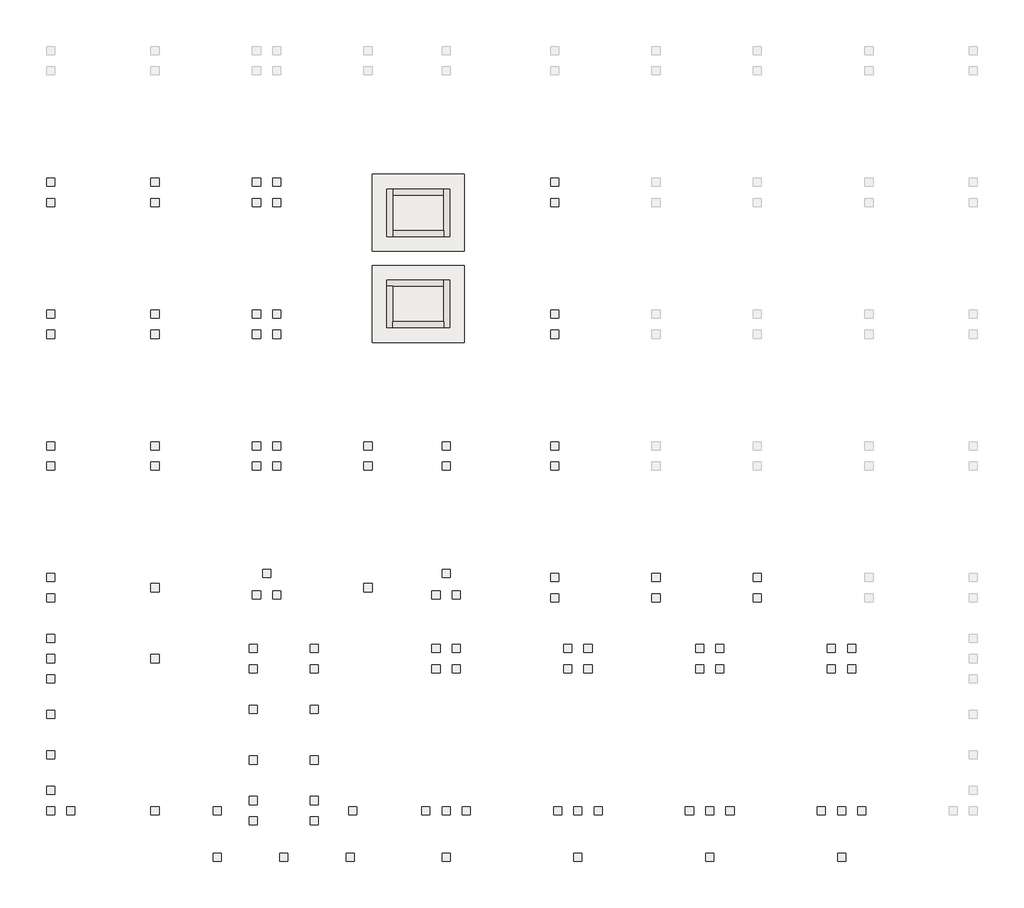
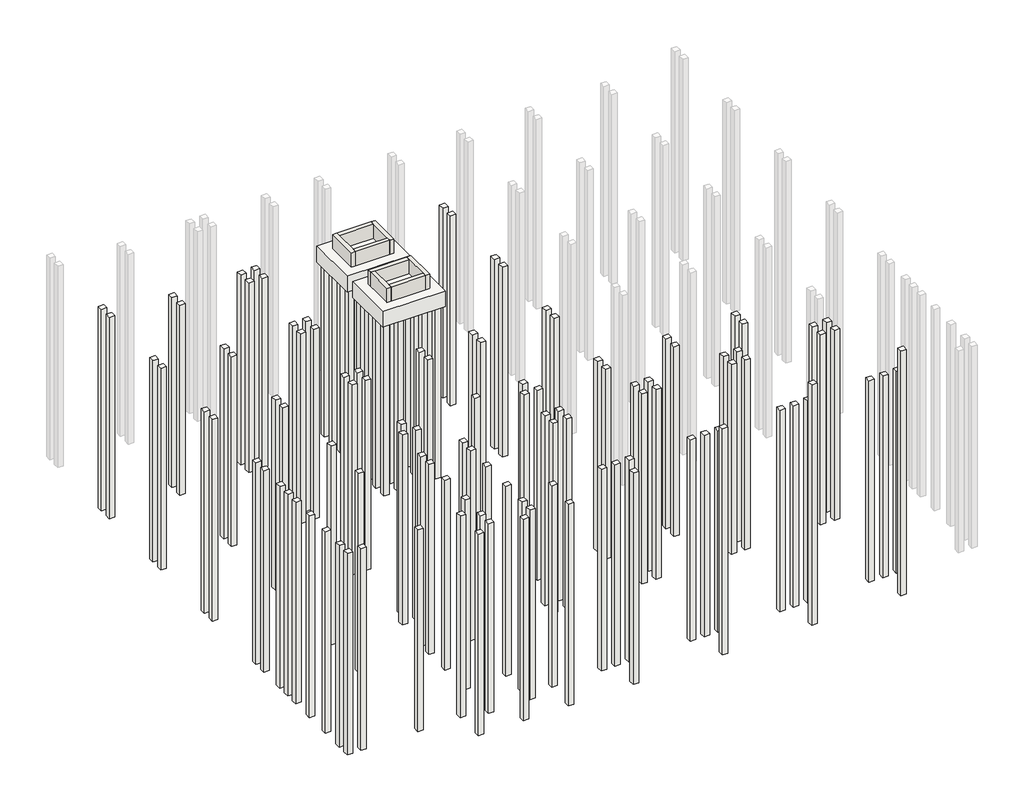
# Not in any storey, part 1 of 2: 143 footings, 8 walls.
"""IFC4 building model written with IfcOpenShell, lengths in millimetres."""

import ifcopenshell
import ifcopenshell.guid

model = None  # the IFC model being written
_history = None  # IfcOwnerHistory: only IFC2X3 demands one
_inside = {}  # id of a spatial element -> (the spatial element, [elements in it])
_under = {}  # id of a project, library or spatial element -> (it, [spatial elements below it])
_declared = {}  # id of a project -> (the project, [libraries it declares])
_typed = {}  # id of a type object -> (the type object, [elements of that type])
_made_of = {}  # id of a material, layer set ... -> (it, [elements and type objects made of it])


def new_model(schema):
    """Start an empty IFC model of exactly this schema.

    Asked for "IFC4X3", IfcOpenShell would pick the latest addendum, in which some entities
    have other attributes; the version numbers below select the first issue.
    IFC2X3 requires an IfcOwnerHistory on every rooted entity: one is made here for all.
    """
    global model, _history
    if schema == "IFC4X3":
        model = ifcopenshell.file(schema_version=(4, 3, 0, 0))
    else:
        model = ifcopenshell.file(schema=schema)
    _inside.clear()
    _under.clear()
    _declared.clear()
    _typed.clear()
    _made_of.clear()
    _history = None
    if model.schema == "IFC2X3":
        org = make("IfcOrganization", Name="unknown")
        user = make(
            "IfcPersonAndOrganization",
            ThePerson=make("IfcPerson", FamilyName="unknown"),
            TheOrganization=org,
        )
        app = make(
            "IfcApplication",
            ApplicationDeveloper=org,
            Version="unknown",
            ApplicationFullName="unknown",
            ApplicationIdentifier="unknown",
        )
        _history = make(
            "IfcOwnerHistory",
            OwningUser=user,
            OwningApplication=app,
            ChangeAction="ADDED",
            CreationDate=0,
        )
    return model


def make(cls, **values):
    """One entity of the class cls with the attributes given. An attribute that is None is left unset."""
    return model.create_entity(
        cls, **{name: value for name, value in values.items() if value is not None}
    )


def rooted(cls, **values):
    """An entity with a GlobalId (a new one), such as an element, a storey or a relation."""
    return make(cls, GlobalId=ifcopenshell.guid.new(), OwnerHistory=_history, **values)


def si_unit(unit_type, name, prefix=None):
    """IfcSIUnit, for example si_unit("LENGTHUNIT", "METRE", prefix="MILLI")."""
    return make("IfcSIUnit", UnitType=unit_type, Prefix=prefix, Name=name)


def assignment(units):
    """IfcUnitAssignment: the units of a project."""
    return None if units is None else make("IfcUnitAssignment", Units=units)


def point(xyz):
    """IfcCartesianPoint."""
    return None if xyz is None else make("IfcCartesianPoint", Coordinates=xyz)


def direction(xyz):
    """IfcDirection."""
    return None if xyz is None else make("IfcDirection", DirectionRatios=xyz)


def frame(location, z_axis=None, x_axis=None):
    """IfcAxis2Placement3D, a coordinate frame: its origin and axes. An axis left out is left unset."""
    return make(
        "IfcAxis2Placement3D",
        Location=point(location),
        Axis=direction(z_axis),
        RefDirection=direction(x_axis),
    )


def origin():
    """The frame at (0, 0, 0) with its axes left unset."""
    return frame((0.0, 0.0, 0.0))


def place(relative_to, where):
    """IfcLocalPlacement: puts the frame where relative to a parent placement (None: the world)."""
    return make(
        "IfcLocalPlacement", PlacementRelTo=relative_to, RelativePlacement=where
    )


def context(
    kind, dimensions, precision=None, world=None, true_north=None, identifier=None
):
    """IfcGeometricRepresentationContext, for example the 3D "Model" context."""
    return make(
        "IfcGeometricRepresentationContext",
        ContextIdentifier=identifier,
        ContextType=kind,
        CoordinateSpaceDimension=dimensions,
        Precision=precision,
        WorldCoordinateSystem=world,
        TrueNorth=true_north,
    )


def project(units=None, contexts=None):
    """IfcProject with its units and contexts."""
    return rooted(
        "IfcProject",
        Name="project",
        RepresentationContexts=contexts,
        UnitsInContext=assignment(units),
    )


def spatial(cls, under=None, at=None, **own):
    """A site, building, storey or space (cls), placed at a placement, below another one or the project."""
    s = rooted(cls, ObjectPlacement=at, **own)
    if under is not None:
        _under.setdefault(under.id(), (under, []))[1].append(s)
    return s


def polyline(points):
    """IfcPolyline through the points."""
    return make("IfcPolyline", Points=[point(p) for p in points])


def outline(outer, holes=None, kind="AREA"):
    """IfcArbitraryClosedProfileDef: a profile drawn as a closed curve; with holes, ...WithVoids."""
    if holes is None:
        return make("IfcArbitraryClosedProfileDef", ProfileType=kind, OuterCurve=outer)
    return make(
        "IfcArbitraryProfileDefWithVoids",
        ProfileType=kind,
        OuterCurve=outer,
        InnerCurves=holes,
    )


def extrude(swept, where, along, depth):
    """IfcExtrudedAreaSolid: the profile swept, set in the frame where, extruded along a direction by depth."""
    return make(
        "IfcExtrudedAreaSolid",
        SweptArea=swept,
        Position=where,
        ExtrudedDirection=direction(along),
        Depth=depth,
    )


def faces_of(points, faces, orient=None, outer=None):
    """IfcFace entities. A face is a list of loops; a loop is a list of indices into points, from 0.

    orient and outer hold one flag for each loop. By default every Orientation is true, the
    first loop of a face is its IfcFaceOuterBound and the others are IfcFaceBound.
    """
    made = []
    for i, loops in enumerate(faces):
        bounds = []
        for j, loop in enumerate(loops):
            is_outer = j == 0 if outer is None else outer[i][j]
            bounds.append(
                make(
                    "IfcFaceOuterBound" if is_outer else "IfcFaceBound",
                    Bound=make("IfcPolyLoop", Polygon=[points[k] for k in loop]),
                    Orientation=True if orient is None else orient[i][j],
                )
            )
        made.append(make("IfcFace", Bounds=bounds))
    return made


def faceted_brep(points, faces, orient=None, outer=None, voids=None):
    """IfcFacetedBrep: a solid bounded by flat faces; with voids (closed shells), ...WithVoids."""
    shared = [point(p) for p in points]
    hull = make("IfcClosedShell", CfsFaces=faces_of(shared, faces, orient, outer))
    if voids is None:
        return make("IfcFacetedBrep", Outer=hull)
    return make(
        "IfcFacetedBrepWithVoids",
        Outer=hull,
        Voids=[
            make(cls, CfsFaces=faces_of(shared, fs, o, b)) for cls, fs, o, b in voids
        ],
    )


def shape(context_of_items, identifier, shape_type, items):
    """IfcShapeRepresentation: the items that make up one representation, for example the "Body"."""
    return make(
        "IfcShapeRepresentation",
        ContextOfItems=context_of_items,
        RepresentationIdentifier=identifier,
        RepresentationType=shape_type,
        Items=items,
    )


def source(mapping_origin, context_of_items, identifier, shape_type, items):
    """IfcRepresentationMap: a shape defined once, which mapped items show again and again."""
    return make(
        "IfcRepresentationMap",
        MappingOrigin=mapping_origin,
        MappedRepresentation=shape(context_of_items, identifier, shape_type, items),
    )


def transform(
    local_origin,
    x_axis=None,
    y_axis=None,
    z_axis=None,
    scale=None,
    scale2=None,
    scale3=None,
    uniform=True,
):
    """IfcCartesianTransformationOperator3D, or its non-uniform kind. x_axis, y_axis, z_axis: its Axis1, 2, 3."""
    if uniform:
        return make(
            "IfcCartesianTransformationOperator3D",
            Axis1=direction(x_axis),
            Axis2=direction(y_axis),
            LocalOrigin=point(local_origin),
            Scale=scale,
            Axis3=direction(z_axis),
        )
    return make(
        "IfcCartesianTransformationOperator3DnonUniform",
        Axis1=direction(x_axis),
        Axis2=direction(y_axis),
        LocalOrigin=point(local_origin),
        Scale=scale,
        Axis3=direction(z_axis),
        Scale2=scale2,
        Scale3=scale3,
    )


def mapped(mapping_source, mapping_target):
    """IfcMappedItem: shows the shape of a source again, moved by a transform."""
    return make(
        "IfcMappedItem", MappingSource=mapping_source, MappingTarget=mapping_target
    )


def made_of(thing, what):
    """Note that an element or type object is made of a material, layer set ...; save() writes the relation."""
    if what is not None:
        _made_of.setdefault(what.id(), (what, []))[1].append(thing)
    return thing


def element(
    cls,
    number,
    at=None,
    inside=None,
    cuts=None,
    type_object=None,
    material=None,
    context=None,
    identifier="Body",
    shape_type=None,
    held_by="IfcProductDefinitionShape",
    body=None,
    shapes=None,
    **own,
):
    """One element of the class cls, such as IfcWall. Its Tag is "e" and its number.

    at: its placement. inside: the storey or other place that contains it. cuts: it is an
    opening in that element (IfcRelVoidsElement). A single representation is given by context,
    identifier, shape_type and body (its items); several are given by shapes. held_by: the class
    of the entity that holds the representations. save() writes the other relations.
    """
    e = rooted(cls, Tag="e%d" % number, ObjectPlacement=at, **own)
    if body is not None:
        shapes = [shape(context, identifier, shape_type, body)]
    if shapes is not None:
        e.Representation = make(held_by, Representations=shapes)
    if inside is not None:
        _inside.setdefault(inside.id(), (inside, []))[1].append(e)
    if cuts is not None:
        rooted(
            "IfcRelVoidsElement", RelatingBuildingElement=cuts, RelatedOpeningElement=e
        )
    if type_object is not None:
        _typed.setdefault(type_object.id(), (type_object, []))[1].append(e)
    return made_of(e, material)


def aggregate(whole, parts):
    """IfcRelAggregates: a whole, such as a stair, and the parts it consists of."""
    return rooted("IfcRelAggregates", RelatingObject=whole, RelatedObjects=parts)


def save(model, path):
    """Write the relations noted so far, then the file.

    IfcRelAggregates (storeys below a building ...), IfcRelContainedInSpatialStructure (elements
    in a storey), IfcRelDefinesByType, IfcRelAssociatesMaterial and IfcRelDeclares: one each for
    every whole, place, type object, material and project.
    """
    for whole, parts in _under.values():
        aggregate(whole, parts)
    for where, things in _inside.values():
        rooted(
            "IfcRelContainedInSpatialStructure",
            RelatedElements=things,
            RelatingStructure=where,
        )
    for kind, things in _typed.values():
        rooted("IfcRelDefinesByType", RelatedObjects=things, RelatingType=kind)
    for what, things in _made_of.values():
        rooted("IfcRelAssociatesMaterial", RelatedObjects=things, RelatingMaterial=what)
    for by, libraries in _declared.values():
        rooted("IfcRelDeclares", RelatingContext=by, RelatedDefinitions=libraries)
    model.write(path)


def footing_e3f33549(model_context):
    return source(origin(), model_context, "Body", "SweptSolid", [
        extrude(outline(polyline([(200.0, -200.0), (-200.0, -200.0), (-200.0, 200.0), (200.0, 200.0), (200.0, -200.0)])), frame((0.0, 0.0, -20000.0), z_axis=(0.0, 0.0, 1.0), x_axis=(1.0, 0.0, 0.0)), (0.0, 0.0, 1.0), 15320.0),
    ])


def footing_2462c6b3(model_context):
    return source(origin(), model_context, "Body", "SweptSolid", [
        extrude(outline(polyline([(200.0, -200.0), (-200.0, -200.0), (-200.0, 200.0), (200.0, 200.0), (200.0, -200.0)])), frame((0.0, 0.0, -20000.0), z_axis=(0.0, 0.0, 1.0), x_axis=(1.0, 0.0, 0.0)), (0.0, 0.0, 1.0), 14620.0),
    ])


def footing_4eaa82be(model_context):
    return source(origin(), model_context, "Body", "SweptSolid", [
        extrude(outline(polyline([(200.0, -200.0), (-200.0, -200.0), (-200.0, 200.0), (200.0, 200.0), (200.0, -200.0)])), frame((0.0, 0.0, -20000.0), z_axis=(0.0, 0.0, 1.0), x_axis=(1.0, 0.0, 0.0)), (0.0, 0.0, 1.0), 15520.0),
    ])


def footing_98706cf3(model_context):
    return source(origin(), model_context, "Body", "SweptSolid", [
        extrude(outline(polyline([(200.0, -200.0), (-200.0, -200.0), (-200.0, 200.0), (200.0, 200.0), (200.0, -200.0)])), frame((0.0, 0.0, -20000.0), z_axis=(0.0, 0.0, 1.0), x_axis=(1.0, 0.0, 0.0)), (0.0, 0.0, 1.0), 16280.0),
    ])


def footing_73a1868d(model_context):
    return source(origin(), model_context, "Body", "SweptSolid", [
        extrude(outline(polyline([(200.0, -200.0), (-200.0, -200.0), (-200.0, 200.0), (200.0, 200.0), (200.0, -200.0)])), frame((0.0, 0.0, -20000.0), z_axis=(0.0, 0.0, 1.0), x_axis=(1.0, 0.0, 0.0)), (0.0, 0.0, 1.0), 17400.0),
    ])


def footing_81e4ded3(model_context):
    return source(origin(), model_context, "Body", "SweptSolid", [
        extrude(outline(polyline([(200.0, -200.0), (-200.0, -200.0), (-200.0, 200.0), (200.0, 200.0), (200.0, -200.0)])), frame((0.0, 0.0, -20000.0), z_axis=(0.0, 0.0, 1.0), x_axis=(1.0, 0.0, 0.0)), (0.0, 0.0, 1.0), 18520.0),
    ])


def footing_0d914d5e(model_context):
    return source(origin(), model_context, "Body", "SweptSolid", [
        extrude(outline(polyline([(200.0, -200.0), (-200.0, -200.0), (-200.0, 200.0), (200.0, 200.0), (200.0, -200.0)])), frame((0.0, 0.0, -20000.0), z_axis=(0.0, 0.0, 1.0), x_axis=(1.0, 0.0, 0.0)), (0.0, 0.0, 1.0), 18850.0),
    ])


def footing_443494b9(model_context):
    return source(origin(), model_context, "Body", "SweptSolid", [
        extrude(outline(polyline([(200.0, -200.0), (-200.0, -200.0), (-200.0, 200.0), (200.0, 200.0), (200.0, -200.0)])), frame((0.0, 0.0, -20000.0), z_axis=(0.0, 0.0, 1.0), x_axis=(1.0, 0.0, 0.0)), (0.0, 0.0, 1.0), 13220.0),
    ])


model = new_model("IFC4")

# Units and contexts
model_context = context("Model", 3, world=origin())
ifc_project = project(units=[si_unit("LENGTHUNIT", "METRE", prefix="MILLI")], contexts=[model_context])

# Site, building
site = spatial("IfcSite", under=ifc_project)
building = spatial("IfcBuilding", under=site)

# Footings
placement = place(None, origin())
element("IfcFooting", 1, at=placement, inside=building, context=model_context, shape_type="SweptSolid", body=[
    extrude(outline(polyline([(22350.0, 27600.0), (22350.0, 31400.0), (26900.0, 31400.0), (26900.0, 27600.0), (22350.0, 27600.0)])), frame((0.0, 0.0, -6800.0), z_axis=(0.0, 0.0, 1.0), x_axis=(1.0, 0.0, 0.0)), (0.0, 0.0, 1.0), 1200.0),
])
element("IfcFooting", 2, at=placement, inside=building, context=model_context, shape_type="SweptSolid", body=[
    extrude(outline(polyline([(22350.0, 23100.0), (22350.0, 26900.0), (26900.0, 26900.0), (26900.0, 23100.0), (22350.0, 23100.0)])), frame((0.0, 0.0, -6800.0), z_axis=(0.0, 0.0, 1.0), x_axis=(1.0, 0.0, 0.0)), (0.0, 0.0, 1.0), 1200.0),
])
footing_shape = footing_e3f33549(model_context)
element("IfcFooting", 3, at=placement, inside=building, context=model_context, shape_type="MappedRepresentation", body=[
    mapped(footing_shape, transform((11650.0, 7500.0, 0.0), x_axis=(1.0, 0.0, 0.0), y_axis=(0.0, 1.0, 0.0), z_axis=(0.0, 0.0, 1.0))),
])
element("IfcFooting", 4, at=placement, inside=building, context=model_context, shape_type="MappedRepresentation", body=[
    mapped(footing_shape, transform((11650.0, 11000.0, 0.0), x_axis=(1.0, 0.0, 0.0), y_axis=(0.0, 1.0, 0.0), z_axis=(0.0, 0.0, 1.0))),
])
element("IfcFooting", 5, at=placement, inside=building, context=model_context, shape_type="MappedRepresentation", body=[
    mapped(footing_shape, transform((22150.0, 11000.0, 0.0), x_axis=(1.0, 0.0, 0.0), y_axis=(0.0, 1.0, 0.0), z_axis=(0.0, 0.0, 1.0))),
])
footing_2_shape = footing_2462c6b3(model_context)
element("IfcFooting", 6, at=placement, inside=building, context=model_context, shape_type="MappedRepresentation", body=[
    mapped(footing_2_shape, transform((22150.0, 17000.0, 0.0), x_axis=(1.0, 0.0, 0.0), y_axis=(0.0, 1.0, 0.0), z_axis=(0.0, 0.0, 1.0))),
])
element("IfcFooting", 7, at=placement, inside=building, context=model_context, shape_type="MappedRepresentation", body=[
    mapped(footing_2_shape, transform((22150.0, 18000.0, 0.0), x_axis=(1.0, 0.0, 0.0), y_axis=(0.0, 1.0, 0.0), z_axis=(0.0, 0.0, 1.0))),
])
element("IfcFooting", 8, at=placement, inside=building, context=model_context, shape_type="MappedRepresentation", body=[
    mapped(footing_2_shape, transform((26000.0, 17000.0, 0.0), x_axis=(1.0, 0.0, 0.0), y_axis=(0.0, 1.0, 0.0), z_axis=(0.0, 0.0, 1.0))),
])
element("IfcFooting", 9, at=placement, inside=building, context=model_context, shape_type="MappedRepresentation", body=[
    mapped(footing_2_shape, transform((26000.0, 18000.0, 0.0), x_axis=(1.0, 0.0, 0.0), y_axis=(0.0, 1.0, 0.0), z_axis=(0.0, 0.0, 1.0))),
])
element("IfcFooting", 10, at=placement, inside=building, context=model_context, shape_type="MappedRepresentation", body=[
    mapped(footing_2_shape, transform((11650.0, 17000.0, 0.0), x_axis=(1.0, 0.0, 0.0), y_axis=(0.0, 1.0, 0.0), z_axis=(0.0, 0.0, 1.0))),
])
element("IfcFooting", 11, at=placement, inside=building, context=model_context, shape_type="MappedRepresentation", body=[
    mapped(footing_2_shape, transform((11650.0, 18000.0, 0.0), x_axis=(1.0, 0.0, 0.0), y_axis=(0.0, 1.0, 0.0), z_axis=(0.0, 0.0, 1.0))),
])
element("IfcFooting", 12, at=placement, inside=building, context=model_context, shape_type="MappedRepresentation", body=[
    mapped(footing_2_shape, transform((11650.0, 23500.0, 0.0), x_axis=(1.0, 0.0, 0.0), y_axis=(0.0, 1.0, 0.0), z_axis=(0.0, 0.0, 1.0))),
])
element("IfcFooting", 13, at=placement, inside=building, context=model_context, shape_type="MappedRepresentation", body=[
    mapped(footing_2_shape, transform((11650.0, 24500.0, 0.0), x_axis=(1.0, 0.0, 0.0), y_axis=(0.0, 1.0, 0.0), z_axis=(0.0, 0.0, 1.0))),
])
element("IfcFooting", 14, at=placement, inside=building, context=model_context, shape_type="MappedRepresentation", body=[
    mapped(footing_2_shape, transform((11650.0, 30000.0, 0.0), x_axis=(1.0, 0.0, 0.0), y_axis=(0.0, 1.0, 0.0), z_axis=(0.0, 0.0, 1.0))),
])
element("IfcFooting", 15, at=placement, inside=building, context=model_context, shape_type="MappedRepresentation", body=[
    mapped(footing_2_shape, transform((11650.0, 31000.0, 0.0), x_axis=(1.0, 0.0, 0.0), y_axis=(0.0, 1.0, 0.0), z_axis=(0.0, 0.0, 1.0))),
])
element("IfcFooting", 16, at=placement, inside=building, context=model_context, shape_type="MappedRepresentation", body=[
    mapped(footing_2_shape, transform((31350.0, 10500.0, 0.0), x_axis=(1.0, 0.0, 0.0), y_axis=(0.0, 1.0, 0.0), z_axis=(0.0, 0.0, 1.0))),
])
element("IfcFooting", 17, at=placement, inside=building, context=model_context, shape_type="MappedRepresentation", body=[
    mapped(footing_2_shape, transform((31350.0, 11500.0, 0.0), x_axis=(1.0, 0.0, 0.0), y_axis=(0.0, 1.0, 0.0), z_axis=(0.0, 0.0, 1.0))),
])
element("IfcFooting", 18, at=placement, inside=building, context=model_context, shape_type="MappedRepresentation", body=[
    mapped(footing_2_shape, transform((36350.0, 10500.0, 0.0), x_axis=(1.0, 0.0, 0.0), y_axis=(0.0, 1.0, 0.0), z_axis=(0.0, 0.0, 1.0))),
])
element("IfcFooting", 19, at=placement, inside=building, context=model_context, shape_type="MappedRepresentation", body=[
    mapped(footing_2_shape, transform((36350.0, 11500.0, 0.0), x_axis=(1.0, 0.0, 0.0), y_axis=(0.0, 1.0, 0.0), z_axis=(0.0, 0.0, 1.0))),
])
element("IfcFooting", 20, at=placement, inside=building, context=model_context, shape_type="MappedRepresentation", body=[
    mapped(footing_2_shape, transform((41350.0, 10500.0, 0.0), x_axis=(1.0, 0.0, 0.0), y_axis=(0.0, 1.0, 0.0), z_axis=(0.0, 0.0, 1.0))),
])
element("IfcFooting", 21, at=placement, inside=building, context=model_context, shape_type="MappedRepresentation", body=[
    mapped(footing_2_shape, transform((41350.0, 11500.0, 0.0), x_axis=(1.0, 0.0, 0.0), y_axis=(0.0, 1.0, 0.0), z_axis=(0.0, 0.0, 1.0))),
])
element("IfcFooting", 22, at=placement, inside=building, context=model_context, shape_type="MappedRepresentation", body=[
    mapped(footing_2_shape, transform((46000.0, 7000.0, 0.0), x_axis=(1.0, 0.0, 0.0), y_axis=(0.0, 1.0, 0.0), z_axis=(0.0, 0.0, 1.0))),
])
element("IfcFooting", 23, at=placement, inside=building, context=model_context, shape_type="MappedRepresentation", body=[
    mapped(footing_2_shape, transform((46000.0, 8000.0, 0.0), x_axis=(1.0, 0.0, 0.0), y_axis=(0.0, 1.0, 0.0), z_axis=(0.0, 0.0, 1.0))),
])
element("IfcFooting", 24, at=placement, inside=building, context=model_context, shape_type="MappedRepresentation", body=[
    mapped(footing_2_shape, transform((45000.0, 7000.0, 0.0), x_axis=(1.0, 0.0, 0.0), y_axis=(0.0, 1.0, 0.0), z_axis=(0.0, 0.0, 1.0))),
])
element("IfcFooting", 25, at=placement, inside=building, context=model_context, shape_type="MappedRepresentation", body=[
    mapped(footing_2_shape, transform((45000.0, 8000.0, 0.0), x_axis=(1.0, 0.0, 0.0), y_axis=(0.0, 1.0, 0.0), z_axis=(0.0, 0.0, 1.0))),
])
element("IfcFooting", 26, at=placement, inside=building, context=model_context, shape_type="MappedRepresentation", body=[
    mapped(footing_2_shape, transform((39500.0, 7000.0, 0.0), x_axis=(1.0, 0.0, 0.0), y_axis=(0.0, 1.0, 0.0), z_axis=(0.0, 0.0, 1.0))),
])
element("IfcFooting", 27, at=placement, inside=building, context=model_context, shape_type="MappedRepresentation", body=[
    mapped(footing_2_shape, transform((39500.0, 8000.0, 0.0), x_axis=(1.0, 0.0, 0.0), y_axis=(0.0, 1.0, 0.0), z_axis=(0.0, 0.0, 1.0))),
])
element("IfcFooting", 28, at=placement, inside=building, context=model_context, shape_type="MappedRepresentation", body=[
    mapped(footing_2_shape, transform((38500.0, 7000.0, 0.0), x_axis=(1.0, 0.0, 0.0), y_axis=(0.0, 1.0, 0.0), z_axis=(0.0, 0.0, 1.0))),
])
element("IfcFooting", 29, at=placement, inside=building, context=model_context, shape_type="MappedRepresentation", body=[
    mapped(footing_2_shape, transform((38500.0, 8000.0, 0.0), x_axis=(1.0, 0.0, 0.0), y_axis=(0.0, 1.0, 0.0), z_axis=(0.0, 0.0, 1.0))),
])
element("IfcFooting", 30, at=placement, inside=building, context=model_context, shape_type="MappedRepresentation", body=[
    mapped(footing_2_shape, transform((33000.0, 7000.0, 0.0), x_axis=(1.0, 0.0, 0.0), y_axis=(0.0, 1.0, 0.0), z_axis=(0.0, 0.0, 1.0))),
])
element("IfcFooting", 31, at=placement, inside=building, context=model_context, shape_type="MappedRepresentation", body=[
    mapped(footing_2_shape, transform((33000.0, 8000.0, 0.0), x_axis=(1.0, 0.0, 0.0), y_axis=(0.0, 1.0, 0.0), z_axis=(0.0, 0.0, 1.0))),
])
element("IfcFooting", 32, at=placement, inside=building, context=model_context, shape_type="MappedRepresentation", body=[
    mapped(footing_2_shape, transform((32000.0, 7000.0, 0.0), x_axis=(1.0, 0.0, 0.0), y_axis=(0.0, 1.0, 0.0), z_axis=(0.0, 0.0, 1.0))),
])
element("IfcFooting", 33, at=placement, inside=building, context=model_context, shape_type="MappedRepresentation", body=[
    mapped(footing_2_shape, transform((32000.0, 8000.0, 0.0), x_axis=(1.0, 0.0, 0.0), y_axis=(0.0, 1.0, 0.0), z_axis=(0.0, 0.0, 1.0))),
])
element("IfcFooting", 34, at=placement, inside=building, context=model_context, shape_type="MappedRepresentation", body=[
    mapped(footing_2_shape, transform((26500.0, 7000.0, 0.0), x_axis=(1.0, 0.0, 0.0), y_axis=(0.0, 1.0, 0.0), z_axis=(0.0, 0.0, 1.0))),
])
element("IfcFooting", 35, at=placement, inside=building, context=model_context, shape_type="MappedRepresentation", body=[
    mapped(footing_2_shape, transform((26500.0, 8000.0, 0.0), x_axis=(1.0, 0.0, 0.0), y_axis=(0.0, 1.0, 0.0), z_axis=(0.0, 0.0, 1.0))),
])
element("IfcFooting", 36, at=placement, inside=building, context=model_context, shape_type="MappedRepresentation", body=[
    mapped(footing_2_shape, transform((25500.0, 7000.0, 0.0), x_axis=(1.0, 0.0, 0.0), y_axis=(0.0, 1.0, 0.0), z_axis=(0.0, 0.0, 1.0))),
])
element("IfcFooting", 37, at=placement, inside=building, context=model_context, shape_type="MappedRepresentation", body=[
    mapped(footing_2_shape, transform((25500.0, 8000.0, 0.0), x_axis=(1.0, 0.0, 0.0), y_axis=(0.0, 1.0, 0.0), z_axis=(0.0, 0.0, 1.0))),
])
element("IfcFooting", 38, at=placement, inside=building, context=model_context, shape_type="MappedRepresentation", body=[
    mapped(footing_2_shape, transform((17650.0, 30000.0, 0.0), x_axis=(1.0, 0.0, 0.0), y_axis=(0.0, 1.0, 0.0), z_axis=(0.0, 0.0, 1.0))),
])
element("IfcFooting", 39, at=placement, inside=building, context=model_context, shape_type="MappedRepresentation", body=[
    mapped(footing_2_shape, transform((17650.0, 31000.0, 0.0), x_axis=(1.0, 0.0, 0.0), y_axis=(0.0, 1.0, 0.0), z_axis=(0.0, 0.0, 1.0))),
])
element("IfcFooting", 40, at=placement, inside=building, context=model_context, shape_type="MappedRepresentation", body=[
    mapped(footing_2_shape, transform((16650.0, 30000.0, 0.0), x_axis=(1.0, 0.0, 0.0), y_axis=(0.0, 1.0, 0.0), z_axis=(0.0, 0.0, 1.0))),
])
element("IfcFooting", 41, at=placement, inside=building, context=model_context, shape_type="MappedRepresentation", body=[
    mapped(footing_2_shape, transform((16650.0, 31000.0, 0.0), x_axis=(1.0, 0.0, 0.0), y_axis=(0.0, 1.0, 0.0), z_axis=(0.0, 0.0, 1.0))),
])
element("IfcFooting", 42, at=placement, inside=building, context=model_context, shape_type="MappedRepresentation", body=[
    mapped(footing_2_shape, transform((17650.0, 23500.0, 0.0), x_axis=(1.0, 0.0, 0.0), y_axis=(0.0, 1.0, 0.0), z_axis=(0.0, 0.0, 1.0))),
])
element("IfcFooting", 43, at=placement, inside=building, context=model_context, shape_type="MappedRepresentation", body=[
    mapped(footing_2_shape, transform((17650.0, 24500.0, 0.0), x_axis=(1.0, 0.0, 0.0), y_axis=(0.0, 1.0, 0.0), z_axis=(0.0, 0.0, 1.0))),
])
element("IfcFooting", 44, at=placement, inside=building, context=model_context, shape_type="MappedRepresentation", body=[
    mapped(footing_2_shape, transform((16650.0, 23500.0, 0.0), x_axis=(1.0, 0.0, 0.0), y_axis=(0.0, 1.0, 0.0), z_axis=(0.0, 0.0, 1.0))),
])
element("IfcFooting", 45, at=placement, inside=building, context=model_context, shape_type="MappedRepresentation", body=[
    mapped(footing_2_shape, transform((16650.0, 24500.0, 0.0), x_axis=(1.0, 0.0, 0.0), y_axis=(0.0, 1.0, 0.0), z_axis=(0.0, 0.0, 1.0))),
])
element("IfcFooting", 46, at=placement, inside=building, context=model_context, shape_type="MappedRepresentation", body=[
    mapped(footing_2_shape, transform((17650.0, 17000.0, 0.0), x_axis=(1.0, 0.0, 0.0), y_axis=(0.0, 1.0, 0.0), z_axis=(0.0, 0.0, 1.0))),
])
element("IfcFooting", 47, at=placement, inside=building, context=model_context, shape_type="MappedRepresentation", body=[
    mapped(footing_2_shape, transform((17650.0, 18000.0, 0.0), x_axis=(1.0, 0.0, 0.0), y_axis=(0.0, 1.0, 0.0), z_axis=(0.0, 0.0, 1.0))),
])
element("IfcFooting", 48, at=placement, inside=building, context=model_context, shape_type="MappedRepresentation", body=[
    mapped(footing_2_shape, transform((16650.0, 17000.0, 0.0), x_axis=(1.0, 0.0, 0.0), y_axis=(0.0, 1.0, 0.0), z_axis=(0.0, 0.0, 1.0))),
])
element("IfcFooting", 49, at=placement, inside=building, context=model_context, shape_type="MappedRepresentation", body=[
    mapped(footing_2_shape, transform((16650.0, 18000.0, 0.0), x_axis=(1.0, 0.0, 0.0), y_axis=(0.0, 1.0, 0.0), z_axis=(0.0, 0.0, 1.0))),
])
element("IfcFooting", 50, at=placement, inside=building, context=model_context, shape_type="MappedRepresentation", body=[
    mapped(footing_2_shape, transform((16650.0, 10650.0, 0.0), x_axis=(1.0, 0.0, 0.0), y_axis=(0.0, 1.0, 0.0), z_axis=(0.0, 0.0, 1.0))),
])
element("IfcFooting", 51, at=placement, inside=building, context=model_context, shape_type="MappedRepresentation", body=[
    mapped(footing_2_shape, transform((17650.0, 10650.0, 0.0), x_axis=(1.0, 0.0, 0.0), y_axis=(0.0, 1.0, 0.0), z_axis=(0.0, 0.0, 1.0))),
])
element("IfcFooting", 52, at=placement, inside=building, context=model_context, shape_type="MappedRepresentation", body=[
    mapped(footing_2_shape, transform((17150.0, 11700.0, 0.0), x_axis=(1.0, 0.0, 0.0), y_axis=(0.0, 1.0, 0.0), z_axis=(0.0, 0.0, 1.0))),
])
element("IfcFooting", 53, at=placement, inside=building, context=model_context, shape_type="MappedRepresentation", body=[
    mapped(footing_2_shape, transform((19500.0, 7000.0, 0.0), x_axis=(1.0, 0.0, 0.0), y_axis=(0.0, 1.0, 0.0), z_axis=(0.0, 0.0, 1.0))),
])
element("IfcFooting", 54, at=placement, inside=building, context=model_context, shape_type="MappedRepresentation", body=[
    mapped(footing_2_shape, transform((19500.0, 8000.0, 0.0), x_axis=(1.0, 0.0, 0.0), y_axis=(0.0, 1.0, 0.0), z_axis=(0.0, 0.0, 1.0))),
])
element("IfcFooting", 55, at=placement, inside=building, context=model_context, shape_type="MappedRepresentation", body=[
    mapped(footing_2_shape, transform((16500.0, 7000.0, 0.0), x_axis=(1.0, 0.0, 0.0), y_axis=(0.0, 1.0, 0.0), z_axis=(0.0, 0.0, 1.0))),
])
element("IfcFooting", 56, at=placement, inside=building, context=model_context, shape_type="MappedRepresentation", body=[
    mapped(footing_2_shape, transform((16500.0, 8000.0, 0.0), x_axis=(1.0, 0.0, 0.0), y_axis=(0.0, 1.0, 0.0), z_axis=(0.0, 0.0, 1.0))),
])
element("IfcFooting", 57, at=placement, inside=building, context=model_context, shape_type="MappedRepresentation", body=[
    mapped(footing_2_shape, transform((19500.0, -500.0, 0.0), x_axis=(1.0, 0.0, 0.0), y_axis=(0.0, 1.0, 0.0), z_axis=(0.0, 0.0, 1.0))),
])
element("IfcFooting", 58, at=placement, inside=building, context=model_context, shape_type="MappedRepresentation", body=[
    mapped(footing_2_shape, transform((19500.0, 500.0, 0.0), x_axis=(1.0, 0.0, 0.0), y_axis=(0.0, 1.0, 0.0), z_axis=(0.0, 0.0, 1.0))),
])
element("IfcFooting", 59, at=placement, inside=building, context=model_context, shape_type="MappedRepresentation", body=[
    mapped(footing_2_shape, transform((16500.0, -500.0, 0.0), x_axis=(1.0, 0.0, 0.0), y_axis=(0.0, 1.0, 0.0), z_axis=(0.0, 0.0, 1.0))),
])
element("IfcFooting", 60, at=placement, inside=building, context=model_context, shape_type="MappedRepresentation", body=[
    mapped(footing_2_shape, transform((16500.0, 500.0, 0.0), x_axis=(1.0, 0.0, 0.0), y_axis=(0.0, 1.0, 0.0), z_axis=(0.0, 0.0, 1.0))),
])
element("IfcFooting", 61, at=placement, inside=building, context=model_context, shape_type="MappedRepresentation", body=[
    mapped(footing_2_shape, transform((16500.0, 5000.0, 0.0), x_axis=(1.0, 0.0, 0.0), y_axis=(0.0, 1.0, 0.0), z_axis=(0.0, 0.0, 1.0))),
])
element("IfcFooting", 62, at=placement, inside=building, context=model_context, shape_type="MappedRepresentation", body=[
    mapped(footing_2_shape, transform((19500.0, 5000.0, 0.0), x_axis=(1.0, 0.0, 0.0), y_axis=(0.0, 1.0, 0.0), z_axis=(0.0, 0.0, 1.0))),
])
element("IfcFooting", 63, at=placement, inside=building, context=model_context, shape_type="MappedRepresentation", body=[
    mapped(footing_2_shape, transform((19500.0, 2500.0, 0.0), x_axis=(1.0, 0.0, 0.0), y_axis=(0.0, 1.0, 0.0), z_axis=(0.0, 0.0, 1.0))),
])
element("IfcFooting", 64, at=placement, inside=building, context=model_context, shape_type="MappedRepresentation", body=[
    mapped(footing_2_shape, transform((16500.0, 2500.0, 0.0), x_axis=(1.0, 0.0, 0.0), y_axis=(0.0, 1.0, 0.0), z_axis=(0.0, 0.0, 1.0))),
])
element("IfcFooting", 65, at=placement, inside=building, context=model_context, shape_type="MappedRepresentation", body=[
    mapped(footing_2_shape, transform((25500.0, 10650.0, 0.0), x_axis=(1.0, 0.0, 0.0), y_axis=(0.0, 1.0, 0.0), z_axis=(0.0, 0.0, 1.0))),
])
element("IfcFooting", 66, at=placement, inside=building, context=model_context, shape_type="MappedRepresentation", body=[
    mapped(footing_2_shape, transform((26500.0, 10650.0, 0.0), x_axis=(1.0, 0.0, 0.0), y_axis=(0.0, 1.0, 0.0), z_axis=(0.0, 0.0, 1.0))),
])
element("IfcFooting", 67, at=placement, inside=building, context=model_context, shape_type="MappedRepresentation", body=[
    mapped(footing_2_shape, transform((26000.0, 11700.0, 0.0), x_axis=(1.0, 0.0, 0.0), y_axis=(0.0, 1.0, 0.0), z_axis=(0.0, 0.0, 1.0))),
])
element("IfcFooting", 68, at=placement, inside=building, context=model_context, shape_type="MappedRepresentation", body=[
    mapped(footing_2_shape, transform((31350.0, 17000.0, 0.0), x_axis=(1.0, 0.0, 0.0), y_axis=(0.0, 1.0, 0.0), z_axis=(0.0, 0.0, 1.0))),
])
element("IfcFooting", 69, at=placement, inside=building, context=model_context, shape_type="MappedRepresentation", body=[
    mapped(footing_2_shape, transform((31350.0, 18000.0, 0.0), x_axis=(1.0, 0.0, 0.0), y_axis=(0.0, 1.0, 0.0), z_axis=(0.0, 0.0, 1.0))),
])
element("IfcFooting", 70, at=placement, inside=building, context=model_context, shape_type="MappedRepresentation", body=[
    mapped(footing_2_shape, transform((31350.0, 23500.0, 0.0), x_axis=(1.0, 0.0, 0.0), y_axis=(0.0, 1.0, 0.0), z_axis=(0.0, 0.0, 1.0))),
])
element("IfcFooting", 71, at=placement, inside=building, context=model_context, shape_type="MappedRepresentation", body=[
    mapped(footing_2_shape, transform((31350.0, 24500.0, 0.0), x_axis=(1.0, 0.0, 0.0), y_axis=(0.0, 1.0, 0.0), z_axis=(0.0, 0.0, 1.0))),
])
element("IfcFooting", 72, at=placement, inside=building, context=model_context, shape_type="MappedRepresentation", body=[
    mapped(footing_2_shape, transform((31350.0, 30000.0, 0.0), x_axis=(1.0, 0.0, 0.0), y_axis=(0.0, 1.0, 0.0), z_axis=(0.0, 0.0, 1.0))),
])
element("IfcFooting", 73, at=placement, inside=building, context=model_context, shape_type="MappedRepresentation", body=[
    mapped(footing_2_shape, transform((31350.0, 31000.0, 0.0), x_axis=(1.0, 0.0, 0.0), y_axis=(0.0, 1.0, 0.0), z_axis=(0.0, 0.0, 1.0))),
])
footing_3_shape = footing_4eaa82be(model_context)
element("IfcFooting", 74, at=placement, inside=building, context=model_context, shape_type="MappedRepresentation", body=[
    mapped(footing_3_shape, transform((6500.0, 8500.0, 0.0), x_axis=(1.0, 0.0, 0.0), y_axis=(0.0, 1.0, 0.0), z_axis=(0.0, 0.0, 1.0))),
])
element("IfcFooting", 75, at=placement, inside=building, context=model_context, shape_type="MappedRepresentation", body=[
    mapped(footing_3_shape, transform((6500.0, 7500.0, 0.0), x_axis=(1.0, 0.0, 0.0), y_axis=(0.0, 1.0, 0.0), z_axis=(0.0, 0.0, 1.0))),
])
element("IfcFooting", 76, at=placement, inside=building, context=model_context, shape_type="MappedRepresentation", body=[
    mapped(footing_3_shape, transform((6500.0, 6500.0, 0.0), x_axis=(1.0, 0.0, 0.0), y_axis=(0.0, 1.0, 0.0), z_axis=(0.0, 0.0, 1.0))),
])
element("IfcFooting", 77, at=placement, inside=building, context=model_context, shape_type="MappedRepresentation", body=[
    mapped(footing_3_shape, transform((6500.0, 0.0, 0.0), x_axis=(1.0, 0.0, 0.0), y_axis=(0.0, 1.0, 0.0), z_axis=(0.0, 0.0, 1.0))),
])
element("IfcFooting", 78, at=placement, inside=building, context=model_context, shape_type="MappedRepresentation", body=[
    mapped(footing_3_shape, transform((6500.0, 1000.0, 0.0), x_axis=(1.0, 0.0, 0.0), y_axis=(0.0, 1.0, 0.0), z_axis=(0.0, 0.0, 1.0))),
])
element("IfcFooting", 79, at=placement, inside=building, context=model_context, shape_type="MappedRepresentation", body=[
    mapped(footing_3_shape, transform((7500.0, 0.0, 0.0), x_axis=(1.0, 0.0, 0.0), y_axis=(0.0, 1.0, 0.0), z_axis=(0.0, 0.0, 1.0))),
])
element("IfcFooting", 80, at=placement, inside=building, context=model_context, shape_type="MappedRepresentation", body=[
    mapped(footing_3_shape, transform((6500.0, 4750.0, 0.0), x_axis=(1.0, 0.0, 0.0), y_axis=(0.0, 1.0, 0.0), z_axis=(0.0, 0.0, 1.0))),
])
element("IfcFooting", 81, at=placement, inside=building, context=model_context, shape_type="MappedRepresentation", body=[
    mapped(footing_3_shape, transform((6500.0, 2750.0, 0.0), x_axis=(1.0, 0.0, 0.0), y_axis=(0.0, 1.0, 0.0), z_axis=(0.0, 0.0, 1.0))),
])
element("IfcFooting", 82, at=placement, inside=building, context=model_context, shape_type="MappedRepresentation", body=[
    mapped(footing_3_shape, transform((14725.0, 0.0, 0.0), x_axis=(1.0, 0.0, 0.0), y_axis=(0.0, 1.0, 0.0), z_axis=(0.0, 0.0, 1.0))),
])
element("IfcFooting", 83, at=placement, inside=building, context=model_context, shape_type="MappedRepresentation", body=[
    mapped(footing_3_shape, transform((11650.0, 0.0, 0.0), x_axis=(1.0, 0.0, 0.0), y_axis=(0.0, 1.0, 0.0), z_axis=(0.0, 0.0, 1.0))),
])
element("IfcFooting", 84, at=placement, inside=building, context=model_context, shape_type="MappedRepresentation", body=[
    mapped(footing_3_shape, transform((45500.0, 0.0, 0.0), x_axis=(1.0, 0.0, 0.0), y_axis=(0.0, 1.0, 0.0), z_axis=(0.0, 0.0, 1.0))),
])
element("IfcFooting", 85, at=placement, inside=building, context=model_context, shape_type="MappedRepresentation", body=[
    mapped(footing_3_shape, transform((46500.0, 0.0, 0.0), x_axis=(1.0, 0.0, 0.0), y_axis=(0.0, 1.0, 0.0), z_axis=(0.0, 0.0, 1.0))),
])
element("IfcFooting", 86, at=placement, inside=building, context=model_context, shape_type="MappedRepresentation", body=[
    mapped(footing_3_shape, transform((44500.0, 0.0, 0.0), x_axis=(1.0, 0.0, 0.0), y_axis=(0.0, 1.0, 0.0), z_axis=(0.0, 0.0, 1.0))),
])
element("IfcFooting", 87, at=placement, inside=building, context=model_context, shape_type="MappedRepresentation", body=[
    mapped(footing_3_shape, transform((39000.0, 0.0, 0.0), x_axis=(1.0, 0.0, 0.0), y_axis=(0.0, 1.0, 0.0), z_axis=(0.0, 0.0, 1.0))),
])
element("IfcFooting", 88, at=placement, inside=building, context=model_context, shape_type="MappedRepresentation", body=[
    mapped(footing_3_shape, transform((40000.0, 0.0, 0.0), x_axis=(1.0, 0.0, 0.0), y_axis=(0.0, 1.0, 0.0), z_axis=(0.0, 0.0, 1.0))),
])
element("IfcFooting", 89, at=placement, inside=building, context=model_context, shape_type="MappedRepresentation", body=[
    mapped(footing_3_shape, transform((38000.0, 0.0, 0.0), x_axis=(1.0, 0.0, 0.0), y_axis=(0.0, 1.0, 0.0), z_axis=(0.0, 0.0, 1.0))),
])
element("IfcFooting", 90, at=placement, inside=building, context=model_context, shape_type="MappedRepresentation", body=[
    mapped(footing_3_shape, transform((32500.0, 0.0, 0.0), x_axis=(1.0, 0.0, 0.0), y_axis=(0.0, 1.0, 0.0), z_axis=(0.0, 0.0, 1.0))),
])
element("IfcFooting", 91, at=placement, inside=building, context=model_context, shape_type="MappedRepresentation", body=[
    mapped(footing_3_shape, transform((33500.0, 0.0, 0.0), x_axis=(1.0, 0.0, 0.0), y_axis=(0.0, 1.0, 0.0), z_axis=(0.0, 0.0, 1.0))),
])
element("IfcFooting", 92, at=placement, inside=building, context=model_context, shape_type="MappedRepresentation", body=[
    mapped(footing_3_shape, transform((31500.0, 0.0, 0.0), x_axis=(1.0, 0.0, 0.0), y_axis=(0.0, 1.0, 0.0), z_axis=(0.0, 0.0, 1.0))),
])
element("IfcFooting", 93, at=placement, inside=building, context=model_context, shape_type="MappedRepresentation", body=[
    mapped(footing_3_shape, transform((26000.0, 0.0, 0.0), x_axis=(1.0, 0.0, 0.0), y_axis=(0.0, 1.0, 0.0), z_axis=(0.0, 0.0, 1.0))),
])
element("IfcFooting", 94, at=placement, inside=building, context=model_context, shape_type="MappedRepresentation", body=[
    mapped(footing_3_shape, transform((27000.0, 0.0, 0.0), x_axis=(1.0, 0.0, 0.0), y_axis=(0.0, 1.0, 0.0), z_axis=(0.0, 0.0, 1.0))),
])
element("IfcFooting", 95, at=placement, inside=building, context=model_context, shape_type="MappedRepresentation", body=[
    mapped(footing_3_shape, transform((25000.0, 0.0, 0.0), x_axis=(1.0, 0.0, 0.0), y_axis=(0.0, 1.0, 0.0), z_axis=(0.0, 0.0, 1.0))),
])
element("IfcFooting", 96, at=placement, inside=building, context=model_context, shape_type="MappedRepresentation", body=[
    mapped(footing_3_shape, transform((21400.0, 0.0, 0.0), x_axis=(1.0, 0.0, 0.0), y_axis=(0.0, 1.0, 0.0), z_axis=(0.0, 0.0, 1.0))),
])
element("IfcFooting", 97, at=placement, inside=building, context=model_context, shape_type="MappedRepresentation", body=[
    mapped(footing_3_shape, transform((6500.0, 10500.0, 0.0), x_axis=(1.0, 0.0, 0.0), y_axis=(0.0, 1.0, 0.0), z_axis=(0.0, 0.0, 1.0))),
])
element("IfcFooting", 98, at=placement, inside=building, context=model_context, shape_type="MappedRepresentation", body=[
    mapped(footing_3_shape, transform((6500.0, 11500.0, 0.0), x_axis=(1.0, 0.0, 0.0), y_axis=(0.0, 1.0, 0.0), z_axis=(0.0, 0.0, 1.0))),
])
element("IfcFooting", 99, at=placement, inside=building, context=model_context, shape_type="MappedRepresentation", body=[
    mapped(footing_3_shape, transform((6500.0, 17000.0, 0.0), x_axis=(1.0, 0.0, 0.0), y_axis=(0.0, 1.0, 0.0), z_axis=(0.0, 0.0, 1.0))),
])
element("IfcFooting", 100, at=placement, inside=building, context=model_context, shape_type="MappedRepresentation", body=[
    mapped(footing_3_shape, transform((6500.0, 18000.0, 0.0), x_axis=(1.0, 0.0, 0.0), y_axis=(0.0, 1.0, 0.0), z_axis=(0.0, 0.0, 1.0))),
])
element("IfcFooting", 101, at=placement, inside=building, context=model_context, shape_type="MappedRepresentation", body=[
    mapped(footing_3_shape, transform((6500.0, 23500.0, 0.0), x_axis=(1.0, 0.0, 0.0), y_axis=(0.0, 1.0, 0.0), z_axis=(0.0, 0.0, 1.0))),
])
element("IfcFooting", 102, at=placement, inside=building, context=model_context, shape_type="MappedRepresentation", body=[
    mapped(footing_3_shape, transform((6500.0, 24500.0, 0.0), x_axis=(1.0, 0.0, 0.0), y_axis=(0.0, 1.0, 0.0), z_axis=(0.0, 0.0, 1.0))),
])
element("IfcFooting", 103, at=placement, inside=building, context=model_context, shape_type="MappedRepresentation", body=[
    mapped(footing_3_shape, transform((6500.0, 30000.0, 0.0), x_axis=(1.0, 0.0, 0.0), y_axis=(0.0, 1.0, 0.0), z_axis=(0.0, 0.0, 1.0))),
])
element("IfcFooting", 104, at=placement, inside=building, context=model_context, shape_type="MappedRepresentation", body=[
    mapped(footing_3_shape, transform((6500.0, 31000.0, 0.0), x_axis=(1.0, 0.0, 0.0), y_axis=(0.0, 1.0, 0.0), z_axis=(0.0, 0.0, 1.0))),
])
element("IfcFooting", 105, at=placement, inside=building, context=model_context, shape_type="MappedRepresentation", body=[
    mapped(footing_3_shape, transform((14725.0, -2300.0, 0.0), x_axis=(1.0, 0.0, 0.0), y_axis=(0.0, 1.0, 0.0), z_axis=(0.0, 0.0, 1.0))),
])
element("IfcFooting", 106, at=placement, inside=building, context=model_context, shape_type="MappedRepresentation", body=[
    mapped(footing_3_shape, transform((21275.0, -2300.0, 0.0), x_axis=(1.0, 0.0, 0.0), y_axis=(0.0, 1.0, 0.0), z_axis=(0.0, 0.0, 1.0))),
])
element("IfcFooting", 107, at=placement, inside=building, context=model_context, shape_type="MappedRepresentation", body=[
    mapped(footing_3_shape, transform((18000.0, -2300.0, 0.0), x_axis=(1.0, 0.0, 0.0), y_axis=(0.0, 1.0, 0.0), z_axis=(0.0, 0.0, 1.0))),
])
footing_4_shape = footing_98706cf3(model_context)
element("IfcFooting", 108, at=placement, inside=building, context=model_context, shape_type="MappedRepresentation", body=[
    mapped(footing_4_shape, transform((26000.0, -2300.0, 0.0), x_axis=(1.0, 0.0, 0.0), y_axis=(0.0, 1.0, 0.0), z_axis=(0.0, 0.0, 1.0))),
])
footing_5_shape = footing_73a1868d(model_context)
element("IfcFooting", 109, at=placement, inside=building, context=model_context, shape_type="MappedRepresentation", body=[
    mapped(footing_5_shape, transform((32500.0, -2300.0, 0.0), x_axis=(1.0, 0.0, 0.0), y_axis=(0.0, 1.0, 0.0), z_axis=(0.0, 0.0, 1.0))),
])
footing_6_shape = footing_81e4ded3(model_context)
element("IfcFooting", 110, at=placement, inside=building, context=model_context, shape_type="MappedRepresentation", body=[
    mapped(footing_6_shape, transform((39000.0, -2300.0, 0.0), x_axis=(1.0, 0.0, 0.0), y_axis=(0.0, 1.0, 0.0), z_axis=(0.0, 0.0, 1.0))),
])
footing_7_shape = footing_0d914d5e(model_context)
element("IfcFooting", 111, at=placement, inside=building, context=model_context, shape_type="MappedRepresentation", body=[
    mapped(footing_7_shape, transform((45500.0, -2300.0, 0.0), x_axis=(1.0, 0.0, 0.0), y_axis=(0.0, 1.0, 0.0), z_axis=(0.0, 0.0, 1.0))),
])
footing_8_shape = footing_443494b9(model_context)
element("IfcFooting", 112, at=placement, inside=building, context=model_context, shape_type="MappedRepresentation", body=[
    mapped(footing_8_shape, transform((23750.0, 31000.0, 0.0), x_axis=(1.0, 0.0, 0.0), y_axis=(0.0, 1.0, 0.0), z_axis=(0.0, 0.0, 1.0))),
])
element("IfcFooting", 113, at=placement, inside=building, context=model_context, shape_type="MappedRepresentation", body=[
    mapped(footing_8_shape, transform((23750.0, 29000.0, 0.0), x_axis=(1.0, 0.0, 0.0), y_axis=(0.0, 1.0, 0.0), z_axis=(0.0, 0.0, 1.0))),
])
element("IfcFooting", 114, at=placement, inside=building, context=model_context, shape_type="MappedRepresentation", body=[
    mapped(footing_8_shape, transform((22750.0, 29000.0, 0.0), x_axis=(1.0, 0.0, 0.0), y_axis=(0.0, 1.0, 0.0), z_axis=(0.0, 0.0, 1.0))),
])
element("IfcFooting", 115, at=placement, inside=building, context=model_context, shape_type="MappedRepresentation", body=[
    mapped(footing_8_shape, transform((22750.0, 31000.0, 0.0), x_axis=(1.0, 0.0, 0.0), y_axis=(0.0, 1.0, 0.0), z_axis=(0.0, 0.0, 1.0))),
])
element("IfcFooting", 116, at=placement, inside=building, context=model_context, shape_type="MappedRepresentation", body=[
    mapped(footing_8_shape, transform((23750.0, 30000.0, 0.0), x_axis=(1.0, 0.0, 0.0), y_axis=(0.0, 1.0, 0.0), z_axis=(0.0, 0.0, 1.0))),
])
element("IfcFooting", 117, at=placement, inside=building, context=model_context, shape_type="MappedRepresentation", body=[
    mapped(footing_8_shape, transform((22750.0, 30000.0, 0.0), x_axis=(1.0, 0.0, 0.0), y_axis=(0.0, 1.0, 0.0), z_axis=(0.0, 0.0, 1.0))),
])
element("IfcFooting", 118, at=placement, inside=building, context=model_context, shape_type="MappedRepresentation", body=[
    mapped(footing_8_shape, transform((23750.0, 28000.0, 0.0), x_axis=(1.0, 0.0, 0.0), y_axis=(0.0, 1.0, 0.0), z_axis=(0.0, 0.0, 1.0))),
])
element("IfcFooting", 119, at=placement, inside=building, context=model_context, shape_type="MappedRepresentation", body=[
    mapped(footing_8_shape, transform((22750.0, 28000.0, 0.0), x_axis=(1.0, 0.0, 0.0), y_axis=(0.0, 1.0, 0.0), z_axis=(0.0, 0.0, 1.0))),
])
element("IfcFooting", 120, at=placement, inside=building, context=model_context, shape_type="MappedRepresentation", body=[
    mapped(footing_8_shape, transform((26500.0, 31000.0, 0.0), x_axis=(1.0, 0.0, 0.0), y_axis=(0.0, 1.0, 0.0), z_axis=(0.0, 0.0, 1.0))),
])
element("IfcFooting", 121, at=placement, inside=building, context=model_context, shape_type="MappedRepresentation", body=[
    mapped(footing_8_shape, transform((26500.0, 29000.0, 0.0), x_axis=(1.0, 0.0, 0.0), y_axis=(0.0, 1.0, 0.0), z_axis=(0.0, 0.0, 1.0))),
])
element("IfcFooting", 122, at=placement, inside=building, context=model_context, shape_type="MappedRepresentation", body=[
    mapped(footing_8_shape, transform((25500.0, 29000.0, 0.0), x_axis=(1.0, 0.0, 0.0), y_axis=(0.0, 1.0, 0.0), z_axis=(0.0, 0.0, 1.0))),
])
element("IfcFooting", 123, at=placement, inside=building, context=model_context, shape_type="MappedRepresentation", body=[
    mapped(footing_8_shape, transform((25500.0, 31000.0, 0.0), x_axis=(1.0, 0.0, 0.0), y_axis=(0.0, 1.0, 0.0), z_axis=(0.0, 0.0, 1.0))),
])
element("IfcFooting", 124, at=placement, inside=building, context=model_context, shape_type="MappedRepresentation", body=[
    mapped(footing_8_shape, transform((26500.0, 30000.0, 0.0), x_axis=(1.0, 0.0, 0.0), y_axis=(0.0, 1.0, 0.0), z_axis=(0.0, 0.0, 1.0))),
])
element("IfcFooting", 125, at=placement, inside=building, context=model_context, shape_type="MappedRepresentation", body=[
    mapped(footing_8_shape, transform((25500.0, 30000.0, 0.0), x_axis=(1.0, 0.0, 0.0), y_axis=(0.0, 1.0, 0.0), z_axis=(0.0, 0.0, 1.0))),
])
element("IfcFooting", 126, at=placement, inside=building, context=model_context, shape_type="MappedRepresentation", body=[
    mapped(footing_8_shape, transform((26500.0, 28000.0, 0.0), x_axis=(1.0, 0.0, 0.0), y_axis=(0.0, 1.0, 0.0), z_axis=(0.0, 0.0, 1.0))),
])
element("IfcFooting", 127, at=placement, inside=building, context=model_context, shape_type="MappedRepresentation", body=[
    mapped(footing_8_shape, transform((25500.0, 28000.0, 0.0), x_axis=(1.0, 0.0, 0.0), y_axis=(0.0, 1.0, 0.0), z_axis=(0.0, 0.0, 1.0))),
])
element("IfcFooting", 128, at=placement, inside=building, context=model_context, shape_type="MappedRepresentation", body=[
    mapped(footing_8_shape, transform((23750.0, 26500.0, 0.0), x_axis=(1.0, 0.0, 0.0), y_axis=(0.0, 1.0, 0.0), z_axis=(0.0, 0.0, 1.0))),
])
element("IfcFooting", 129, at=placement, inside=building, context=model_context, shape_type="MappedRepresentation", body=[
    mapped(footing_8_shape, transform((23750.0, 24500.0, 0.0), x_axis=(1.0, 0.0, 0.0), y_axis=(0.0, 1.0, 0.0), z_axis=(0.0, 0.0, 1.0))),
])
element("IfcFooting", 130, at=placement, inside=building, context=model_context, shape_type="MappedRepresentation", body=[
    mapped(footing_8_shape, transform((22750.0, 24500.0, 0.0), x_axis=(1.0, 0.0, 0.0), y_axis=(0.0, 1.0, 0.0), z_axis=(0.0, 0.0, 1.0))),
])
element("IfcFooting", 131, at=placement, inside=building, context=model_context, shape_type="MappedRepresentation", body=[
    mapped(footing_8_shape, transform((22750.0, 26500.0, 0.0), x_axis=(1.0, 0.0, 0.0), y_axis=(0.0, 1.0, 0.0), z_axis=(0.0, 0.0, 1.0))),
])
element("IfcFooting", 132, at=placement, inside=building, context=model_context, shape_type="MappedRepresentation", body=[
    mapped(footing_8_shape, transform((23750.0, 25500.0, 0.0), x_axis=(1.0, 0.0, 0.0), y_axis=(0.0, 1.0, 0.0), z_axis=(0.0, 0.0, 1.0))),
])
element("IfcFooting", 133, at=placement, inside=building, context=model_context, shape_type="MappedRepresentation", body=[
    mapped(footing_8_shape, transform((22750.0, 25500.0, 0.0), x_axis=(1.0, 0.0, 0.0), y_axis=(0.0, 1.0, 0.0), z_axis=(0.0, 0.0, 1.0))),
])
element("IfcFooting", 134, at=placement, inside=building, context=model_context, shape_type="MappedRepresentation", body=[
    mapped(footing_8_shape, transform((23750.0, 23500.0, 0.0), x_axis=(1.0, 0.0, 0.0), y_axis=(0.0, 1.0, 0.0), z_axis=(0.0, 0.0, 1.0))),
])
element("IfcFooting", 135, at=placement, inside=building, context=model_context, shape_type="MappedRepresentation", body=[
    mapped(footing_8_shape, transform((22750.0, 23500.0, 0.0), x_axis=(1.0, 0.0, 0.0), y_axis=(0.0, 1.0, 0.0), z_axis=(0.0, 0.0, 1.0))),
])
element("IfcFooting", 136, at=placement, inside=building, context=model_context, shape_type="MappedRepresentation", body=[
    mapped(footing_8_shape, transform((26500.0, 26500.0, 0.0), x_axis=(1.0, 0.0, 0.0), y_axis=(0.0, 1.0, 0.0), z_axis=(0.0, 0.0, 1.0))),
])
element("IfcFooting", 137, at=placement, inside=building, context=model_context, shape_type="MappedRepresentation", body=[
    mapped(footing_8_shape, transform((26500.0, 24500.0, 0.0), x_axis=(1.0, 0.0, 0.0), y_axis=(0.0, 1.0, 0.0), z_axis=(0.0, 0.0, 1.0))),
])
element("IfcFooting", 138, at=placement, inside=building, context=model_context, shape_type="MappedRepresentation", body=[
    mapped(footing_8_shape, transform((25500.0, 24500.0, 0.0), x_axis=(1.0, 0.0, 0.0), y_axis=(0.0, 1.0, 0.0), z_axis=(0.0, 0.0, 1.0))),
])
element("IfcFooting", 139, at=placement, inside=building, context=model_context, shape_type="MappedRepresentation", body=[
    mapped(footing_8_shape, transform((25500.0, 26500.0, 0.0), x_axis=(1.0, 0.0, 0.0), y_axis=(0.0, 1.0, 0.0), z_axis=(0.0, 0.0, 1.0))),
])
element("IfcFooting", 140, at=placement, inside=building, context=model_context, shape_type="MappedRepresentation", body=[
    mapped(footing_8_shape, transform((26500.0, 25500.0, 0.0), x_axis=(1.0, 0.0, 0.0), y_axis=(0.0, 1.0, 0.0), z_axis=(0.0, 0.0, 1.0))),
])
element("IfcFooting", 141, at=placement, inside=building, context=model_context, shape_type="MappedRepresentation", body=[
    mapped(footing_8_shape, transform((25500.0, 25500.0, 0.0), x_axis=(1.0, 0.0, 0.0), y_axis=(0.0, 1.0, 0.0), z_axis=(0.0, 0.0, 1.0))),
])
element("IfcFooting", 142, at=placement, inside=building, context=model_context, shape_type="MappedRepresentation", body=[
    mapped(footing_8_shape, transform((26500.0, 23500.0, 0.0), x_axis=(1.0, 0.0, 0.0), y_axis=(0.0, 1.0, 0.0), z_axis=(0.0, 0.0, 1.0))),
])
element("IfcFooting", 143, at=placement, inside=building, context=model_context, shape_type="MappedRepresentation", body=[
    mapped(footing_8_shape, transform((25500.0, 23500.0, 0.0), x_axis=(1.0, 0.0, 0.0), y_axis=(0.0, 1.0, 0.0), z_axis=(0.0, 0.0, 1.0))),
])

# Walls
element("IfcWall", 144, at=placement, inside=building, context=model_context, shape_type="SweptSolid", body=[
    extrude(outline(polyline([(23375.0, 30675.0), (25875.0, 30675.0), (25875.0, 30375.0), (23375.0, 30375.0), (23375.0, 30675.0)])), frame((0.0, 0.0, -5600.0), z_axis=(0.0, 0.0, 1.0), x_axis=(1.0, 0.0, 0.0)), (0.0, 0.0, 1.0), 1100.0),
])
element("IfcWall", 145, at=placement, inside=building, context=model_context, shape_type="Brep", body=[
    faceted_brep([(23075.0, 30675.0, -5600.0), (23075.0, 28325.0, -5600.0), (23075.0, 28325.0, -4500.0), (23075.0, 30675.0, -4500.0), (23375.0, 30675.0, -5600.0), (23375.0, 30675.0, -4500.0), (23375.0, 30375.0, -4500.0), (23375.0, 28625.0, -4500.0), (23375.0, 28325.0, -4500.0), (23375.0, 28325.0, -5600.0), (23375.0, 28625.0, -5600.0), (23375.0, 30375.0, -5600.0)], [[[0, 1, 2, 3]], [[4, 5, 6, 7, 8, 9, 10, 11]], [[1, 0, 4, 11, 10, 9]], [[2, 1, 9, 8]], [[3, 2, 8, 7, 6, 5]], [[0, 3, 5, 4]]]),
])
element("IfcWall", 146, at=placement, inside=building, context=model_context, shape_type="SweptSolid", body=[
    extrude(outline(polyline([(25875.0, 28325.0), (23375.0, 28325.0), (23375.0, 28625.0), (25875.0, 28625.0), (25875.0, 28325.0)])), frame((0.0, 0.0, -5600.0), z_axis=(0.0, 0.0, 1.0), x_axis=(1.0, 0.0, 0.0)), (0.0, 0.0, 1.0), 1100.0),
])
element("IfcWall", 147, at=placement, inside=building, context=model_context, shape_type="Brep", body=[
    faceted_brep([(26175.0, 23825.0, -5600.0), (26175.0, 26175.0, -5600.0), (26175.0, 26175.0, -4500.0), (26175.0, 23825.0, -4500.0), (25875.0, 23825.0, -5600.0), (25875.0, 23825.0, -4500.0), (25875.0, 24125.0, -4500.0), (25875.0, 25875.0, -4500.0), (25875.0, 26175.0, -4500.0), (25875.0, 26175.0, -5600.0), (25875.0, 25875.0, -5600.0), (25875.0, 24125.0, -5600.0)], [[[0, 1, 2, 3]], [[4, 5, 6, 7, 8, 9, 10, 11]], [[1, 0, 4, 11, 10, 9]], [[3, 2, 8, 7, 6, 5]], [[0, 3, 5, 4]], [[2, 1, 9, 8]]]),
])
element("IfcWall", 148, at=placement, inside=building, context=model_context, shape_type="Brep", body=[
    faceted_brep([(25875.0, 26175.0, -5600.0), (23075.0, 26175.0, -5600.0), (23075.0, 26175.0, -4500.0), (25875.0, 26175.0, -4500.0), (25875.0, 25875.0, -5600.0), (25875.0, 25875.0, -4500.0), (23375.0, 25875.0, -4500.0), (23075.0, 25875.0, -4500.0), (23075.0, 25875.0, -5600.0), (23375.0, 25875.0, -5600.0)], [[[0, 1, 2, 3]], [[4, 5, 6, 7, 8, 9]], [[1, 0, 4, 9, 8]], [[3, 2, 7, 6, 5]], [[2, 1, 8, 7]], [[0, 3, 5, 4]]]),
])
element("IfcWall", 149, at=placement, inside=building, context=model_context, shape_type="Brep", body=[
    faceted_brep([(23075.0, 25875.0, -5600.0), (23075.0, 23825.0, -5600.0), (23075.0, 23825.0, -4500.0), (23075.0, 25875.0, -4500.0), (23375.0, 25875.0, -5600.0), (23375.0, 25875.0, -4500.0), (23375.0, 24125.0, -4500.0), (23375.0, 23825.0, -4500.0), (23375.0, 23825.0, -5600.0), (23375.0, 24125.0, -5600.0)], [[[0, 1, 2, 3]], [[4, 5, 6, 7, 8, 9]], [[1, 0, 4, 9, 8]], [[3, 2, 7, 6, 5]], [[2, 1, 8, 7]], [[0, 3, 5, 4]]]),
])
element("IfcWall", 150, at=placement, inside=building, context=model_context, shape_type="SweptSolid", body=[
    extrude(outline(polyline([(25875.0, 23825.0), (23375.0, 23825.0), (23375.0, 24125.0), (25875.0, 24125.0), (25875.0, 23825.0)])), frame((0.0, 0.0, -5600.0), z_axis=(0.0, 0.0, 1.0), x_axis=(1.0, 0.0, 0.0)), (0.0, 0.0, 1.0), 1100.0),
])
element("IfcWall", 151, at=placement, inside=building, context=model_context, shape_type="Brep", body=[
    faceted_brep([(26175.0, 28325.0, -5600.0), (26175.0, 30675.0, -5600.0), (26175.0, 30675.0, -4500.0), (26175.0, 28325.0, -4500.0), (25875.0, 28325.0, -5600.0), (25875.0, 28325.0, -4500.0), (25875.0, 28625.0, -4500.0), (25875.0, 30375.0, -4500.0), (25875.0, 30675.0, -4500.0), (25875.0, 30675.0, -5600.0), (25875.0, 30375.0, -5600.0), (25875.0, 28625.0, -5600.0)], [[[0, 1, 2, 3]], [[4, 5, 6, 7, 8, 9, 10, 11]], [[1, 0, 4, 11, 10, 9]], [[2, 1, 9, 8]], [[3, 2, 8, 7, 6, 5]], [[0, 3, 5, 4]]]),
])

save(model, "model.ifc")

# Revit data of these elements
# Type "NLRS_16_SFO_LB_funderingspoer meerpaals beton ihwg-MMBC-SH_gen_rsf : funderingspoer beton ihwg_gen__lift bxlxh 3800x4550x1200"
#   IfcExportAs = "IfcFootingType"
#   Type Comments = "liftpoer 3800x4550x1200"
#   Model = " "
#   Manufacturer = " "
#   Description = "liftpoer 3800x4550x1200"
#   Assembly Code = "16.13"
#   Width = 3800 mm
#   Rough Height = 1200 mm
#   NLRS_C_lengte = 4550 mm
#   NLRS_C_hoogte = 1200 mm
#   NLRS_C_breedte = 3800 mm
#   Length = 4550 mm
#   Height [instance default] = 1050 mm
#   Foundation Thickness = 1200 mm
#   Depth [instance default] = 150 mm
#   Structural Material = NLRS_f2_beton ihwg_gen_rsf
#   Keynote = ""
